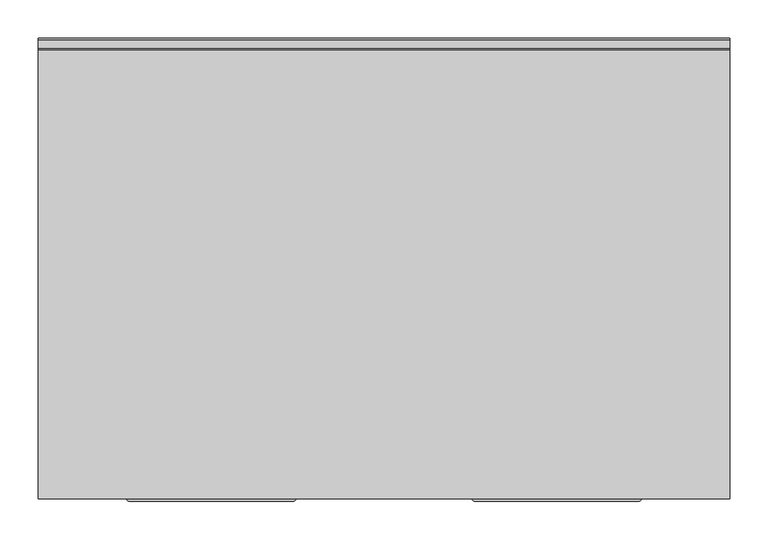
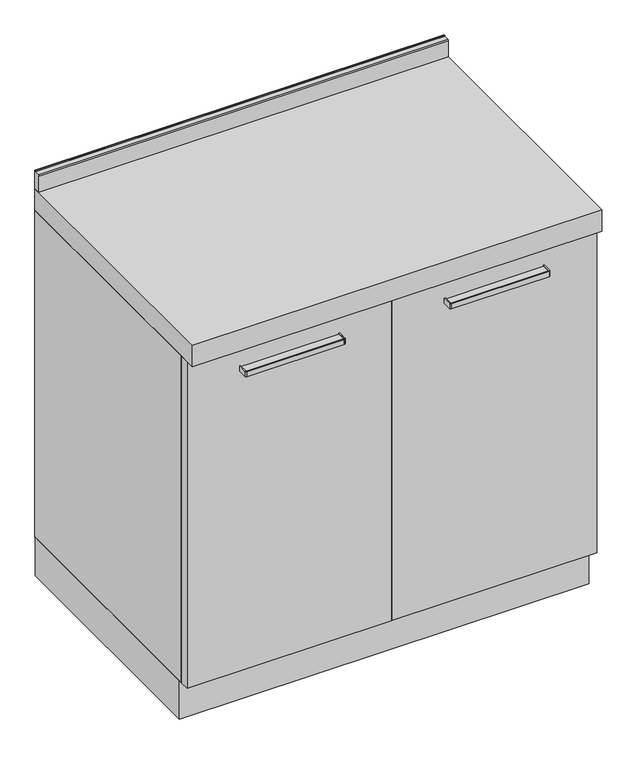
"""IFC4 building model written with IfcOpenShell, lengths in millimetres: furniture geometry, Küchenelement (1) - 2-flg : Küchenschränke."""

from ifc_helpers import new_model, si_unit, point, frame, frame_2d, origin, origin_with_axes, place, context, project, spatial, polyline, circle_curve, trimmed, segment, composite_curve, outline, extrude, source, transform, mapped, element, save


def furniture_8fb8675d(model_context):
    return source(origin(), model_context, "Body", "SweptSolid", [
        extrude(outline(composite_curve([segment(polyline([(161.7003264, -580.0), (377.7003264, -580.0), (377.7003264, -600.5)]), True, "CONTINUOUS"), segment(trimmed(circle_curve(frame_2d((377.2003264, -600.5)), 0.5), [point((377.7003264, -600.5))], [point((377.2003264, -601.0))], False, "CARTESIAN"), True, "CONTINUOUS"), segment(polyline([(377.2003264, -601.0), (162.2003264, -601.0)]), True, "CONTINUOUS"), segment(trimmed(circle_curve(frame_2d((162.2003264, -600.5)), 0.5), [point((162.2003264, -601.0))], [point((161.7003264, -600.5))], False, "CARTESIAN"), True, "CONTINUOUS"), segment(polyline([(161.7003264, -600.5), (161.7003264, -580.0)]), True, "CONTINUOUS")], self_intersect=False)), frame((0.0, 0.0, 789.965389), z_axis=(0.0, 0.0, 1.0), x_axis=(1.0, 0.0, 0.0)), (0.0, 0.0, 1.0), 6.4890959),
        extrude(outline(composite_curve([segment(polyline([(159.7003264, -580.0), (161.7003264, -580.0), (161.7003264, -600.5)]), True, "CONTINUOUS"), segment(trimmed(circle_curve(frame_2d((162.2003264, -600.5)), 0.5), [point((161.7003264, -600.5))], [point((162.2003264, -601.0))], True, "CARTESIAN"), True, "CONTINUOUS"), segment(polyline([(162.2003264, -601.0), (377.2003264, -601.0)]), True, "CONTINUOUS"), segment(trimmed(circle_curve(frame_2d((377.2003264, -600.5)), 0.5), [point((377.2003264, -601.0))], [point((377.7003264, -600.5))], True, "CARTESIAN"), True, "CONTINUOUS"), segment(polyline([(377.7003264, -600.5), (377.7003264, -580.0), (379.7003264, -580.0), (379.7003264, -600.5)]), True, "CONTINUOUS"), segment(trimmed(circle_curve(frame_2d((377.2003264, -600.5)), 2.5), [point((379.7003264, -600.5))], [point((377.2003264, -603.0))], False, "CARTESIAN"), True, "CONTINUOUS"), segment(polyline([(377.2003264, -603.0), (162.2003264, -603.0)]), True, "CONTINUOUS"), segment(trimmed(circle_curve(frame_2d((162.2003264, -600.5)), 2.5), [point((162.2003264, -603.0))], [point((159.7003264, -600.5))], False, "CARTESIAN"), True, "CONTINUOUS"), segment(polyline([(159.7003264, -600.5), (159.7003264, -580.0)]), True, "CONTINUOUS")], self_intersect=False)), frame((0.0, 0.0, 787.2), z_axis=(0.0, 0.0, 1.0), x_axis=(1.0, 0.0, 0.0)), (0.0, 0.0, 1.0), 12.0),
        extrude(outline(composite_curve([segment(polyline([(-288.2996736, -580.0), (-72.2996736, -580.0), (-72.2996736, -600.5)]), True, "CONTINUOUS"), segment(trimmed(circle_curve(frame_2d((-72.7996736, -600.5)), 0.5), [point((-72.2996736, -600.5))], [point((-72.7996736, -601.0))], False, "CARTESIAN"), True, "CONTINUOUS"), segment(polyline([(-72.7996736, -601.0), (-287.7996736, -601.0)]), True, "CONTINUOUS"), segment(trimmed(circle_curve(frame_2d((-287.7996736, -600.5)), 0.5), [point((-287.7996736, -601.0))], [point((-288.2996736, -600.5))], False, "CARTESIAN"), True, "CONTINUOUS"), segment(polyline([(-288.2996736, -600.5), (-288.2996736, -580.0)]), True, "CONTINUOUS")], self_intersect=False)), frame((0.0, 0.0, 789.965389), z_axis=(0.0, 0.0, 1.0), x_axis=(1.0, 0.0, 0.0)), (0.0, 0.0, 1.0), 6.4890959),
        extrude(outline(composite_curve([segment(polyline([(-290.2996736, -580.0), (-288.2996736, -580.0), (-288.2996736, -600.5)]), True, "CONTINUOUS"), segment(trimmed(circle_curve(frame_2d((-287.7996736, -600.5)), 0.5), [point((-288.2996736, -600.5))], [point((-287.7996736, -601.0))], True, "CARTESIAN"), True, "CONTINUOUS"), segment(polyline([(-287.7996736, -601.0), (-72.7996736, -601.0)]), True, "CONTINUOUS"), segment(trimmed(circle_curve(frame_2d((-72.7996736, -600.5)), 0.5), [point((-72.7996736, -601.0))], [point((-72.2996736, -600.5))], True, "CARTESIAN"), True, "CONTINUOUS"), segment(polyline([(-72.2996736, -600.5), (-72.2996736, -580.0), (-70.2996736, -580.0), (-70.2996736, -600.5)]), True, "CONTINUOUS"), segment(trimmed(circle_curve(frame_2d((-72.7996736, -600.5)), 2.5), [point((-70.2996736, -600.5))], [point((-72.7996736, -603.0))], False, "CARTESIAN"), True, "CONTINUOUS"), segment(polyline([(-72.7996736, -603.0), (-287.7996736, -603.0)]), True, "CONTINUOUS"), segment(trimmed(circle_curve(frame_2d((-287.7996736, -600.5)), 2.5), [point((-287.7996736, -603.0))], [point((-290.2996736, -600.5))], False, "CARTESIAN"), True, "CONTINUOUS"), segment(polyline([(-290.2996736, -600.5), (-290.2996736, -580.0)]), True, "CONTINUOUS")], self_intersect=False)), frame((0.0, 0.0, 787.2), z_axis=(0.0, 0.0, 1.0), x_axis=(1.0, 0.0, 0.0)), (0.0, 0.0, 1.0), 12.0),
        extrude(outline(composite_curve([segment(polyline([(0.0, 942.0034681), (0.0, 900.0), (-15.0, 900.0), (-15.0, 938.0)]), True, "CONTINUOUS"), segment(trimmed(circle_curve(frame_2d((-13.0, 938.0)), 2.0), [point((-15.0, 938.0))], [point((-13.0, 940.0))], False, "CARTESIAN"), True, "CONTINUOUS"), segment(polyline([(-13.0, 940.0), (-1.50449, 940.0), (-1.50449, 942.0034681), (0.0, 942.0034681)]), True, "CONTINUOUS")], self_intersect=False)), frame((-405.2996736, 0.0, 0.0), z_axis=(1.0, 0.0, 0.0), x_axis=(0.0, 1.0, 0.0)), (0.0, 0.0, 1.0), 900.0),
        extrude(outline(polyline([(494.7003264, -0.533703), (494.7003264, -550.533703), (-405.2996736, -550.533703), (-405.2996736, -0.533703), (494.7003264, -0.533703)])), origin_with_axes(), (0.0, 0.0, 1.0), 90.0),
        extrude(outline(polyline([(494.7003264, 0.0), (494.7003264, -600.0), (-405.2996736, -600.0), (-405.2996736, 0.0), (494.7003264, 0.0)])), frame((0.0, 0.0, 850.0), z_axis=(0.0, 0.0, 1.0), x_axis=(1.0, 0.0, 0.0)), (0.0, 0.0, 1.0), 50.0),
        extrude(outline(polyline([(43.7003264, -580.0), (-405.2996736, -580.0), (-405.2996736, -558.0), (43.7003264, -558.0), (43.7003264, -580.0)])), frame((0.0, 0.0, 90.0), z_axis=(0.0, 0.0, 1.0), x_axis=(1.0, 0.0, 0.0)), (0.0, 0.0, 1.0), 760.0),
        extrude(outline(polyline([(45.7003264, -580.0), (45.7003264, -558.0), (494.7003264, -558.0), (494.7003264, -580.0), (45.7003264, -580.0)])), frame((0.0, 0.0, 90.0), z_axis=(0.0, 0.0, 1.0), x_axis=(1.0, 0.0, 0.0)), (0.0, 0.0, 1.0), 760.0),
        extrude(outline(polyline([(494.7003264, 0.0), (494.7003264, -558.0), (472.7003264, -558.0), (472.7003264, -22.0), (-383.2996736, -22.0), (-383.2996736, -558.0), (-405.2996736, -558.0), (-405.2996736, 0.0), (494.7003264, 0.0)])), frame((0.0, 0.0, 90.0), z_axis=(0.0, 0.0, 1.0), x_axis=(1.0, 0.0, 0.0)), (0.0, 0.0, 1.0), 760.0),
    ])


if __name__ == "__main__":
    model = new_model("IFC4")
    model_context = context("Model", 3, world=origin())
    ifc_project = project(units=[si_unit("LENGTHUNIT", "METRE", prefix="MILLI")], contexts=[model_context])
    site = spatial("IfcSite", under=ifc_project)
    building = spatial("IfcBuilding", under=site)
    placement = place(None, origin())
    furniture_shape = furniture_8fb8675d(model_context)
    element("IfcFurniture", 1, ObjectType="Küchenelement (1) - 2-flg : Küchenschränke", at=placement, inside=building, context=model_context, shape_type="MappedRepresentation", body=[
        mapped(furniture_shape, transform((0.0, 0.0, 0.0), x_axis=(1.0, 0.0, 0.0), y_axis=(0.0, 1.0, 0.0), z_axis=(0.0, 0.0, 1.0))),
    ])
    save(model, "model.ifc")

# Revit data of these elements
# Type "Küchenelement (1) - 2-flg : Küchenschränke"
#   Länge 1 = 0.1008 m
#   Depth = 0.600 m
#   Height = 0.900 m
#   Width = 0.900 m
#   Obermaterial = Kunststoff
#   Material = Kunststoff
#   Griffmaterial = none
#   Assembly Code = ""
# Element 1 (IfcFurniture, "Küchenelement (1) - 2-flg : Küchenschränke")
#   Materials on its faces: "Kunststoff"
# Materials
#   "Kunststoff": class "Allgemeines", colour RGB 0 0 0, transparency 0, Cost = 0
